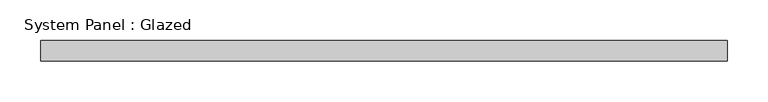
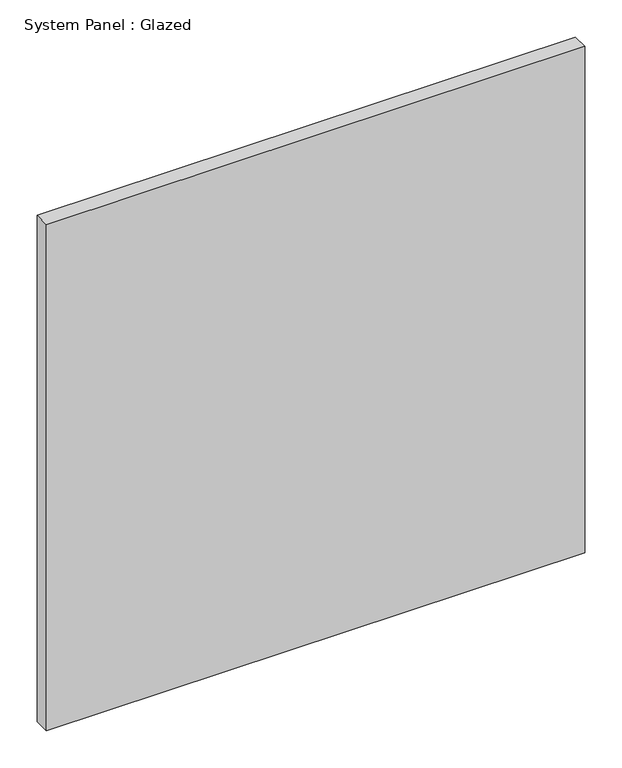
"""IFC4 building model written with IfcOpenShell, lengths in millimetres: plate geometry, System Panel : Glazed."""

from ifc_helpers import new_model, si_unit, origin, origin_with_axes, place, context, project, spatial, polyline, outline, extrude, source, transform, mapped, element, save


def system_panel_glazed_f62d01d8(model_context):
    return source(origin(), model_context, "Body", "SweptSolid", [
        extrude(outline(polyline([(418.9393939, 24.5), (-418.9393939, 24.5), (-418.9393939, 49.5), (418.9393939, 49.5), (418.9393939, 24.5)])), origin_with_axes(), (0.0, 0.0, 1.0), 833.3333333),
    ])


if __name__ == "__main__":
    model = new_model("IFC4")
    model_context = context("Model", 3, world=origin())
    ifc_project = project(units=[si_unit("LENGTHUNIT", "METRE", prefix="MILLI")], contexts=[model_context])
    site = spatial("IfcSite", under=ifc_project)
    building = spatial("IfcBuilding", under=site)
    placement = place(None, origin())
    system_panel_glazed_shape = system_panel_glazed_f62d01d8(model_context)
    element("IfcPlate", 1, ObjectType="System Panel : Glazed", at=placement, inside=building, context=model_context, shape_type="MappedRepresentation", body=[
        mapped(system_panel_glazed_shape, transform((0.0, 0.0, 0.0), x_axis=(1.0, 0.0, 0.0), y_axis=(0.0, 1.0, 0.0), z_axis=(0.0, 0.0, 1.0))),
    ])
    save(model, "model.ifc")

# Revit data of these elements
# Element 1 (IfcPlate, "System Panel : Glazed")
#   Materials on its faces: "Glass"
# Materials
#   "Glass": class "Glass", colour RGB 218 227 224, transparency 0.85, Description = "Soda Lime Glass", Cost = 0
